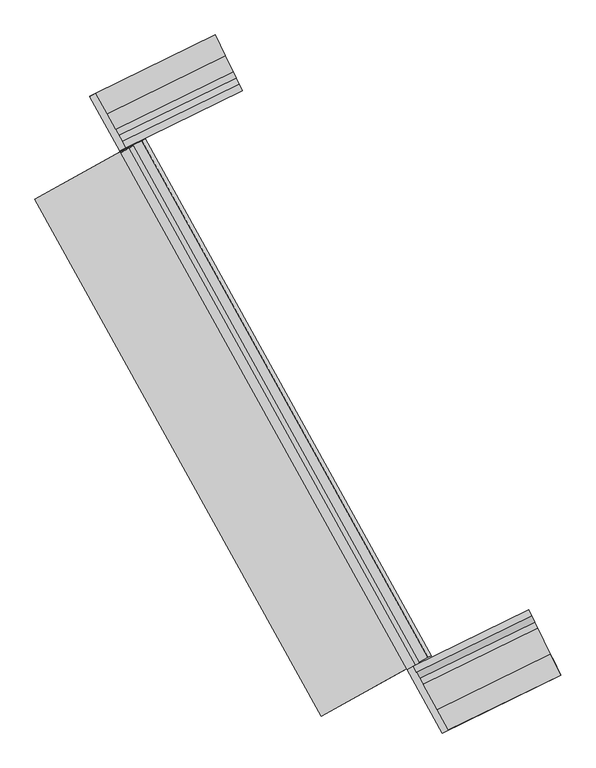
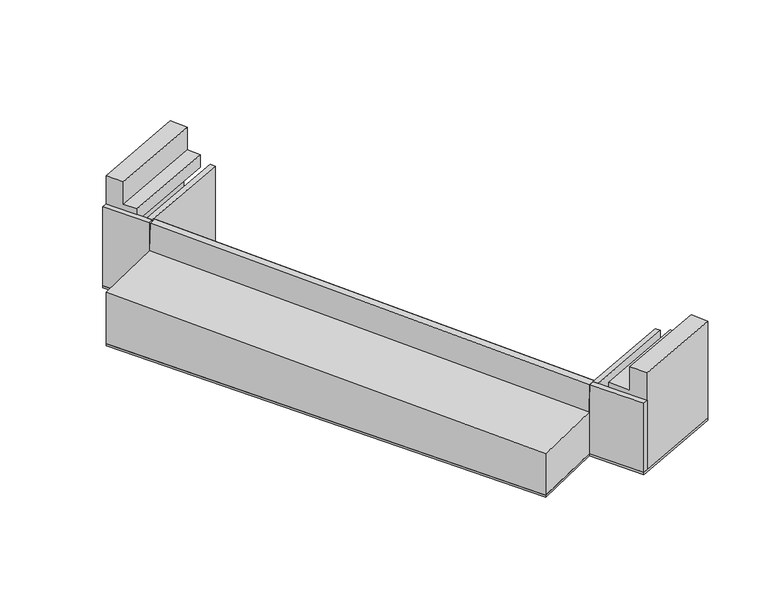
"""IFC4 building model written with IfcOpenShell, lengths in millimetres: beam geometry, KNA_SF_LH_ as4 : KNA_SF_LH_ as4."""

import ifcopenshell
import ifcopenshell.guid

model = None  # the IFC model being written
_history = None  # IfcOwnerHistory: only IFC2X3 demands one
_inside = {}  # id of a spatial element -> (the spatial element, [elements in it])
_under = {}  # id of a project, library or spatial element -> (it, [spatial elements below it])
_declared = {}  # id of a project -> (the project, [libraries it declares])
_typed = {}  # id of a type object -> (the type object, [elements of that type])
_made_of = {}  # id of a material, layer set ... -> (it, [elements and type objects made of it])


def new_model(schema):
    """Start an empty IFC model of exactly this schema.

    Asked for "IFC4X3", IfcOpenShell would pick the latest addendum, in which some entities
    have other attributes; the version numbers below select the first issue.
    IFC2X3 requires an IfcOwnerHistory on every rooted entity: one is made here for all.
    """
    global model, _history
    if schema == "IFC4X3":
        model = ifcopenshell.file(schema_version=(4, 3, 0, 0))
    else:
        model = ifcopenshell.file(schema=schema)
    _inside.clear()
    _under.clear()
    _declared.clear()
    _typed.clear()
    _made_of.clear()
    _history = None
    if model.schema == "IFC2X3":
        org = make("IfcOrganization", Name="unknown")
        user = make(
            "IfcPersonAndOrganization",
            ThePerson=make("IfcPerson", FamilyName="unknown"),
            TheOrganization=org,
        )
        app = make(
            "IfcApplication",
            ApplicationDeveloper=org,
            Version="unknown",
            ApplicationFullName="unknown",
            ApplicationIdentifier="unknown",
        )
        _history = make(
            "IfcOwnerHistory",
            OwningUser=user,
            OwningApplication=app,
            ChangeAction="ADDED",
            CreationDate=0,
        )
    return model


def make(cls, **values):
    """One entity of the class cls with the attributes given. An attribute that is None is left unset."""
    return model.create_entity(
        cls, **{name: value for name, value in values.items() if value is not None}
    )


def rooted(cls, **values):
    """An entity with a GlobalId (a new one), such as an element, a storey or a relation."""
    return make(cls, GlobalId=ifcopenshell.guid.new(), OwnerHistory=_history, **values)


def si_unit(unit_type, name, prefix=None):
    """IfcSIUnit, for example si_unit("LENGTHUNIT", "METRE", prefix="MILLI")."""
    return make("IfcSIUnit", UnitType=unit_type, Prefix=prefix, Name=name)


def assignment(units):
    """IfcUnitAssignment: the units of a project."""
    return None if units is None else make("IfcUnitAssignment", Units=units)


def point(xyz):
    """IfcCartesianPoint."""
    return None if xyz is None else make("IfcCartesianPoint", Coordinates=xyz)


def direction(xyz):
    """IfcDirection."""
    return None if xyz is None else make("IfcDirection", DirectionRatios=xyz)


def frame(location, z_axis=None, x_axis=None):
    """IfcAxis2Placement3D, a coordinate frame: its origin and axes. An axis left out is left unset."""
    return make(
        "IfcAxis2Placement3D",
        Location=point(location),
        Axis=direction(z_axis),
        RefDirection=direction(x_axis),
    )


def origin():
    """The frame at (0, 0, 0) with its axes left unset."""
    return frame((0.0, 0.0, 0.0))


def place(relative_to, where):
    """IfcLocalPlacement: puts the frame where relative to a parent placement (None: the world)."""
    return make(
        "IfcLocalPlacement", PlacementRelTo=relative_to, RelativePlacement=where
    )


def context(
    kind, dimensions, precision=None, world=None, true_north=None, identifier=None
):
    """IfcGeometricRepresentationContext, for example the 3D "Model" context."""
    return make(
        "IfcGeometricRepresentationContext",
        ContextIdentifier=identifier,
        ContextType=kind,
        CoordinateSpaceDimension=dimensions,
        Precision=precision,
        WorldCoordinateSystem=world,
        TrueNorth=true_north,
    )


def project(units=None, contexts=None):
    """IfcProject with its units and contexts."""
    return rooted(
        "IfcProject",
        Name="project",
        RepresentationContexts=contexts,
        UnitsInContext=assignment(units),
    )


def spatial(cls, under=None, at=None, **own):
    """A site, building, storey or space (cls), placed at a placement, below another one or the project."""
    s = rooted(cls, ObjectPlacement=at, **own)
    if under is not None:
        _under.setdefault(under.id(), (under, []))[1].append(s)
    return s


def polyline(points):
    """IfcPolyline through the points."""
    return make("IfcPolyline", Points=[point(p) for p in points])


def outline(outer, holes=None, kind="AREA"):
    """IfcArbitraryClosedProfileDef: a profile drawn as a closed curve; with holes, ...WithVoids."""
    if holes is None:
        return make("IfcArbitraryClosedProfileDef", ProfileType=kind, OuterCurve=outer)
    return make(
        "IfcArbitraryProfileDefWithVoids",
        ProfileType=kind,
        OuterCurve=outer,
        InnerCurves=holes,
    )


def extrude(swept, where, along, depth):
    """IfcExtrudedAreaSolid: the profile swept, set in the frame where, extruded along a direction by depth."""
    return make(
        "IfcExtrudedAreaSolid",
        SweptArea=swept,
        Position=where,
        ExtrudedDirection=direction(along),
        Depth=depth,
    )


def faces_of(points, faces, orient=None, outer=None):
    """IfcFace entities. A face is a list of loops; a loop is a list of indices into points, from 0.

    orient and outer hold one flag for each loop. By default every Orientation is true, the
    first loop of a face is its IfcFaceOuterBound and the others are IfcFaceBound.
    """
    made = []
    for i, loops in enumerate(faces):
        bounds = []
        for j, loop in enumerate(loops):
            is_outer = j == 0 if outer is None else outer[i][j]
            bounds.append(
                make(
                    "IfcFaceOuterBound" if is_outer else "IfcFaceBound",
                    Bound=make("IfcPolyLoop", Polygon=[points[k] for k in loop]),
                    Orientation=True if orient is None else orient[i][j],
                )
            )
        made.append(make("IfcFace", Bounds=bounds))
    return made


def faceted_brep(points, faces, orient=None, outer=None, voids=None):
    """IfcFacetedBrep: a solid bounded by flat faces; with voids (closed shells), ...WithVoids."""
    shared = [point(p) for p in points]
    hull = make("IfcClosedShell", CfsFaces=faces_of(shared, faces, orient, outer))
    if voids is None:
        return make("IfcFacetedBrep", Outer=hull)
    return make(
        "IfcFacetedBrepWithVoids",
        Outer=hull,
        Voids=[
            make(cls, CfsFaces=faces_of(shared, fs, o, b)) for cls, fs, o, b in voids
        ],
    )


def shape(context_of_items, identifier, shape_type, items):
    """IfcShapeRepresentation: the items that make up one representation, for example the "Body"."""
    return make(
        "IfcShapeRepresentation",
        ContextOfItems=context_of_items,
        RepresentationIdentifier=identifier,
        RepresentationType=shape_type,
        Items=items,
    )


def source(mapping_origin, context_of_items, identifier, shape_type, items):
    """IfcRepresentationMap: a shape defined once, which mapped items show again and again."""
    return make(
        "IfcRepresentationMap",
        MappingOrigin=mapping_origin,
        MappedRepresentation=shape(context_of_items, identifier, shape_type, items),
    )


def transform(
    local_origin,
    x_axis=None,
    y_axis=None,
    z_axis=None,
    scale=None,
    scale2=None,
    scale3=None,
    uniform=True,
):
    """IfcCartesianTransformationOperator3D, or its non-uniform kind. x_axis, y_axis, z_axis: its Axis1, 2, 3."""
    if uniform:
        return make(
            "IfcCartesianTransformationOperator3D",
            Axis1=direction(x_axis),
            Axis2=direction(y_axis),
            LocalOrigin=point(local_origin),
            Scale=scale,
            Axis3=direction(z_axis),
        )
    return make(
        "IfcCartesianTransformationOperator3DnonUniform",
        Axis1=direction(x_axis),
        Axis2=direction(y_axis),
        LocalOrigin=point(local_origin),
        Scale=scale,
        Axis3=direction(z_axis),
        Scale2=scale2,
        Scale3=scale3,
    )


def mapped(mapping_source, mapping_target):
    """IfcMappedItem: shows the shape of a source again, moved by a transform."""
    return make(
        "IfcMappedItem", MappingSource=mapping_source, MappingTarget=mapping_target
    )


def made_of(thing, what):
    """Note that an element or type object is made of a material, layer set ...; save() writes the relation."""
    if what is not None:
        _made_of.setdefault(what.id(), (what, []))[1].append(thing)
    return thing


def element(
    cls,
    number,
    at=None,
    inside=None,
    cuts=None,
    type_object=None,
    material=None,
    context=None,
    identifier="Body",
    shape_type=None,
    held_by="IfcProductDefinitionShape",
    body=None,
    shapes=None,
    **own,
):
    """One element of the class cls, such as IfcWall. Its Tag is "e" and its number.

    at: its placement. inside: the storey or other place that contains it. cuts: it is an
    opening in that element (IfcRelVoidsElement). A single representation is given by context,
    identifier, shape_type and body (its items); several are given by shapes. held_by: the class
    of the entity that holds the representations. save() writes the other relations.
    """
    e = rooted(cls, Tag="e%d" % number, ObjectPlacement=at, **own)
    if body is not None:
        shapes = [shape(context, identifier, shape_type, body)]
    if shapes is not None:
        e.Representation = make(held_by, Representations=shapes)
    if inside is not None:
        _inside.setdefault(inside.id(), (inside, []))[1].append(e)
    if cuts is not None:
        rooted(
            "IfcRelVoidsElement", RelatingBuildingElement=cuts, RelatedOpeningElement=e
        )
    if type_object is not None:
        _typed.setdefault(type_object.id(), (type_object, []))[1].append(e)
    return made_of(e, material)


def aggregate(whole, parts):
    """IfcRelAggregates: a whole, such as a stair, and the parts it consists of."""
    return rooted("IfcRelAggregates", RelatingObject=whole, RelatedObjects=parts)


def save(model, path):
    """Write the relations noted so far, then the file.

    IfcRelAggregates (storeys below a building ...), IfcRelContainedInSpatialStructure (elements
    in a storey), IfcRelDefinesByType, IfcRelAssociatesMaterial and IfcRelDeclares: one each for
    every whole, place, type object, material and project.
    """
    for whole, parts in _under.values():
        aggregate(whole, parts)
    for where, things in _inside.values():
        rooted(
            "IfcRelContainedInSpatialStructure",
            RelatedElements=things,
            RelatingStructure=where,
        )
    for kind, things in _typed.values():
        rooted("IfcRelDefinesByType", RelatedObjects=things, RelatingType=kind)
    for what, things in _made_of.values():
        rooted("IfcRelAssociatesMaterial", RelatedObjects=things, RelatingMaterial=what)
    for by, libraries in _declared.values():
        rooted("IfcRelDeclares", RelatingContext=by, RelatedDefinitions=libraries)
    model.write(path)


def beam_7a07aaa9(model_context):
    return source(origin(), model_context, "Body", "SolidModel", [
        extrude(outline(polyline([(167091.7082562, -18021.7193168), (167737.9138009, -19188.9731537), (167606.6820669, -19261.6245955), (166960.4765222, -18094.3707585), (167091.7082562, -18021.7193168)])), frame((0.0, 0.0, 3750.0), z_axis=(0.0, 0.0, 1.0), x_axis=(1.0, 0.0, 0.0)), (0.0, 0.0, 1.0), 2379.7765645),
        faceted_brep([(167091.7082562, -18021.7193168, 6983.0), (169656.5093094, -16768.0418857, 6983.0), (169656.5093094, -16768.0418857, 3750.0), (167091.7082562, -18021.7193168, 3750.0), (170241.6533999, -17965.1426251, 3750.0), (167737.9138009, -19188.9731537, 3750.0), (170241.6533999, -17965.1426251, 6137.1387333), (167737.9138009, -19188.9731537, 6137.1387333), (170175.7814349, -17830.3803002, 6140.6887751), (167665.1679085, -19057.5708116, 6140.6887751), (170175.7814349, -17830.3803002, 5690.6887751), (167665.1679085, -19057.5708116, 5690.6887751), (170109.9094699, -17695.6179753, 5540.6887751), (167592.4220161, -18926.1684696, 5540.6887751), (170109.9094699, -17695.6179753, 4050.0), (167592.4220161, -18926.1684696, 4050.0), (169832.1678829, -17127.4080856, 4050.0), (167285.6973026, -18372.1255623, 4050.0), (169832.1678829, -17127.4080856, 5927.8308621), (167285.6973026, -18372.1255623, 5927.8308621), (170044.0375048, -17560.8556503, 5927.8308621), (167519.6761237, -18794.7661275, 5927.8308621), (170044.0375048, -17560.8556503, 6297.8308621), (167519.6761237, -18794.7661275, 6297.8308621), (169876.0825262, -17217.2496355, 6306.8824698), (167334.1945642, -18459.7271237, 6306.8824698), (169876.0825262, -17217.2496355, 6983.0), (167334.1945642, -18459.7271237, 6983.0)], [[[0, 1, 2, 3]], [[3, 2, 4, 5]], [[5, 4, 6, 7]], [[7, 6, 8, 9]], [[9, 8, 10, 11]], [[11, 10, 12, 13]], [[13, 12, 14, 15]], [[15, 14, 16, 17]], [[17, 16, 18, 19]], [[19, 18, 20, 21]], [[21, 20, 22, 23]], [[23, 22, 24, 25]], [[25, 24, 26, 27]], [[1, 0, 27, 26]], [[2, 1, 26, 24, 22, 20, 18, 16, 14, 12, 10, 8, 6, 4]], [[0, 3, 5, 7, 9, 11, 13, 15, 17, 19, 21, 23, 25, 27]]]),
        extrude(outline(polyline([(174533.0129405, -31772.7928374), (173777.5718569, -30408.2246893), (173908.8035909, -30335.5732475), (174667.9504634, -31706.8352354), (174533.0129405, -31772.7928374)])), frame((0.0, 0.0, 3750.0), z_axis=(0.0, 0.0, 1.0), x_axis=(1.0, 0.0, 0.0)), (0.0, 0.0, 1.0), 2085.7765645),
        faceted_brep([(177080.1600254, -30527.7446845, 6673.0), (177080.1600254, -30527.7446845, 3750.0), (176391.2177768, -29118.2913744, 3750.0), (176391.2177768, -29118.2913744, 5836.7926595), (176457.0897418, -29253.0536994, 5836.7926595), (176457.0897418, -29253.0536994, 5386.7926595), (176522.9617068, -29387.8160243, 5236.7926595), (176522.9617068, -29387.8160243, 4050.0), (176904.5014519, -30168.3784846, 4050.0), (176904.5014519, -30168.3784846, 5609.7345794), (176588.8336719, -29522.5783492, 5609.7345794), (176588.8336719, -29522.5783492, 5975.4700059), (176860.5868086, -30078.5369347, 5960.8243978), (176860.5868086, -30078.5369347, 6673.0), (174425.4641554, -31268.8274285, 6673.0), (174667.9504634, -31706.8352354, 6673.0), (174425.4641554, -31268.8274285, 5960.8243978), (174125.3528042, -30726.7303679, 5975.4700059), (174125.3528042, -30726.7303679, 5609.7345794), (174473.961417, -31356.4289898, 5609.7345794), (174473.961417, -31356.4289898, 4050.0), (174052.6069118, -30595.3280258, 4050.0), (174052.6069118, -30595.3280258, 5236.7926595), (173979.8610194, -30463.9256838, 5386.7926595), (173979.8610194, -30463.9256838, 5836.7926595), (173907.115127, -30332.5233417, 5836.7926595), (173907.115127, -30332.5233417, 3750.0), (174667.9504634, -31706.8352354, 3750.0)], [[[0, 1, 2, 3, 4, 5, 6, 7, 8, 9, 10, 11, 12, 13]], [[0, 13, 14, 15]], [[13, 12, 16, 14]], [[12, 11, 17, 16]], [[11, 10, 18, 17]], [[10, 9, 19, 18]], [[9, 8, 20, 19]], [[8, 7, 21, 20]], [[7, 6, 22, 21]], [[6, 5, 23, 22]], [[5, 4, 24, 23]], [[4, 3, 25, 24]], [[3, 2, 26, 25]], [[2, 1, 27, 26]], [[1, 0, 15, 27]], [[15, 14, 16, 17, 18, 19, 20, 21, 22, 23, 24, 25, 26, 27]]]),
        extrude(outline(polyline([(0.0, -369.0), (-80.0000001, -394.0), (-300.0, -394.0), (-300.0000001, -764.0), (-400.0, -764.0), (-400.0, -834.0), (-600.0000001, -834.0), (-600.0, 0.0), (0.0, 0.0), (0.0, -369.0)])), frame((174293.1490859, -30100.7303617, 5002.0), z_axis=(-0.4842131855684572, 0.8746438395921066, 0.023146161349657045), x_axis=(0.8748782267130657, 0.48434294505381387, 0.0)), (0.0, 0.0, 1.0), 12701.8901994),
        extrude(outline(polyline([(-773.0, 0.0), (773.0, 0.0), (773.0, -12698.4872577), (-479.0, -12698.4872577), (-773.0, 0.0)])), frame((165780.5551576, -20298.8262993, 4523.0), z_axis=(0.8748782267130657, 0.48434294505381387, 0.0), x_axis=(0.0, 0.0, -1.0)), (0.0, 0.0, 1.0), 2700.0),
        extrude(outline(polyline([(165780.5551576, -20298.8262993), (167617.7994337, -19281.7061147), (166956.7707333, -18087.6769188), (169656.5093094, -16768.0418857), (169832.1678829, -17127.4080856), (167690.5098714, -18174.2527563), (174878.7739859, -31158.5561838), (176907.9559703, -30166.6899125), (177083.6145437, -30526.0561123), (174533.0129405, -31772.7928374), (173768.2221498, -30391.3361287), (171930.9778737, -31408.4563133), (165780.5551576, -20298.8262993)])), frame((0.0, 0.0, 3680.0), z_axis=(0.0, 0.0, 1.0), x_axis=(1.0, 0.0, 0.0)), (0.0, 0.0, 1.0), 70.0),
    ])


if __name__ == "__main__":
    model = new_model("IFC4")
    model_context = context("Model", 3, world=origin())
    ifc_project = project(units=[si_unit("LENGTHUNIT", "METRE", prefix="MILLI")], contexts=[model_context])
    site = spatial("IfcSite", under=ifc_project)
    building = spatial("IfcBuilding", under=site)
    placement = place(None, origin())
    beam_shape = beam_7a07aaa9(model_context)
    element("IfcBeam", 1, ObjectType="KNA_SF_LH_ as4 : KNA_SF_LH_ as4", at=placement, inside=building, context=model_context, shape_type="MappedRepresentation", body=[
        mapped(beam_shape, transform((0.0, 0.0, 0.0), x_axis=(1.0, 0.0, 0.0), y_axis=(0.0, 1.0, 0.0), z_axis=(0.0, 0.0, 1.0))),
    ])
    save(model, "model.ifc")

# Revit data of these elements
# Element 1 (IfcBeam, "KNA_SF_LH_ as4 : KNA_SF_LH_ as4")
#   Materials on its faces: "Beton_Bestaande Constructie", "Beton_In-Situ_Werkvloer"
# Materials
#   "Beton_Bestaande Constructie": class "Concrete", colour RGB 102 102 102, transparency 0, Description = "Beton", Cost = 0
#   "Beton_In-Situ_Werkvloer": class "Concrete", colour RGB 128 128 128, transparency 0, Description = "Beton", Cost = 0
